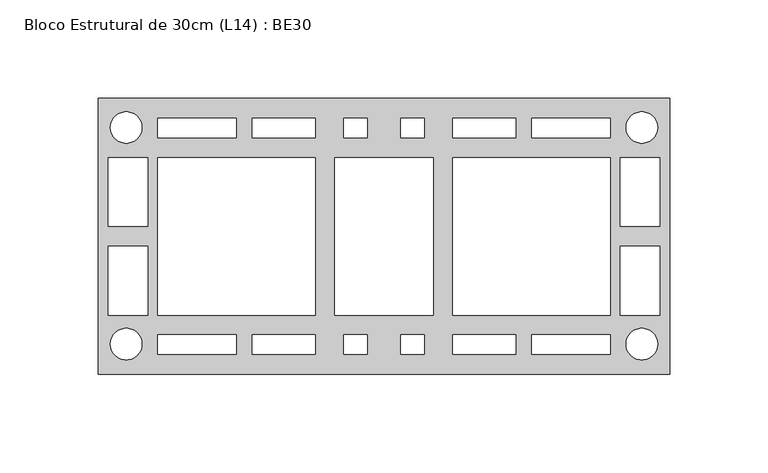
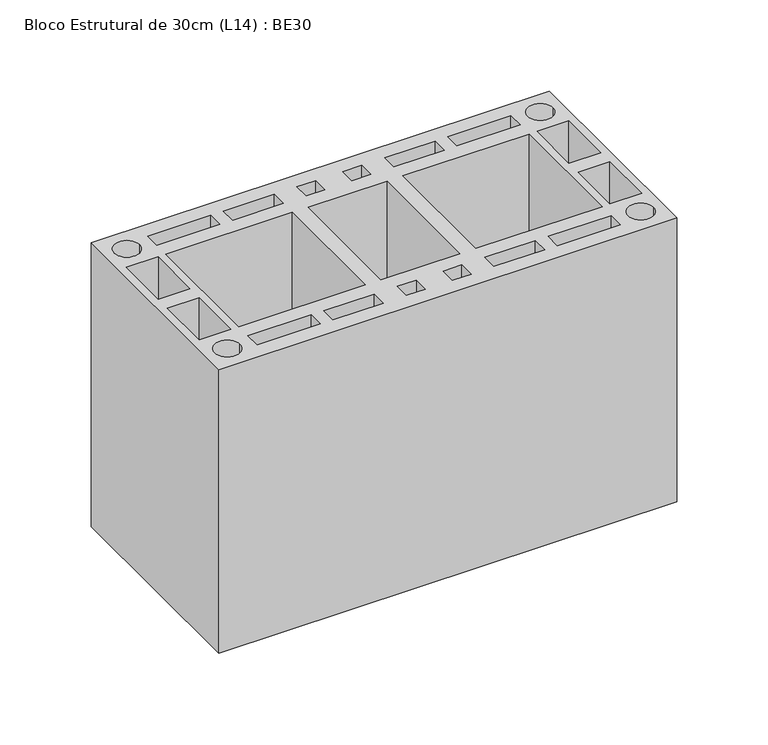
"""IFC4 building model written with IfcOpenShell, lengths in millimetres: proxy geometry, Bloco Estrutural de 30cm (L14) : BE30."""

from ifc_helpers import new_model, si_unit, point, frame_2d, origin, origin_with_axes, place, context, project, spatial, polyline, circle_curve, trimmed, segment, composite_curve, outline, extrude, source, transform, mapped, element, save


def bloco_estrutural_de_30cm_l14_be30_ec04c00f(model_context):
    return source(origin(), model_context, "Body", "SweptSolid", [
        extrude(outline(polyline([(290.0, 0.0), (290.0, -140.0), (0.0, -140.0), (0.0, 0.0), (290.0, 0.0)]), holes=[composite_curve([segment(trimmed(circle_curve(frame_2d((14.1087523, -124.7509514)), 8.0), [point((6.1087523, -124.7509514))], [point((22.1087523, -124.7509514))], True, "CARTESIAN"), True, "CONTINUOUS"), segment(trimmed(circle_curve(frame_2d((14.1087523, -124.7509514)), 8.0), [point((22.1087523, -124.7509514))], [point((6.1087523, -124.7509514))], True, "CARTESIAN"), True, "CONTINUOUS")], self_intersect=False), composite_curve([segment(trimmed(circle_curve(frame_2d((14.1087523, -14.7509514)), 8.0), [point((6.1087523, -14.7509514))], [point((22.1087523, -14.7509514))], True, "CARTESIAN"), True, "CONTINUOUS"), segment(trimmed(circle_curve(frame_2d((14.1087523, -14.7509514)), 8.0), [point((22.1087523, -14.7509514))], [point((6.1087523, -14.7509514))], True, "CARTESIAN"), True, "CONTINUOUS")], self_intersect=False), polyline([(110.0, -110.0), (110.0, -30.0), (30.0, -30.0), (30.0, -110.0), (110.0, -110.0)]), polyline([(170.0, -110.0), (170.0, -30.0), (120.0, -30.0), (120.0, -110.0), (170.0, -110.0)]), polyline([(70.0, -130.0), (70.0, -120.0), (30.0, -120.0), (30.0, -130.0), (70.0, -130.0)]), polyline([(70.0, -20.0), (70.0, -10.0), (30.0, -10.0), (30.0, -20.0), (70.0, -20.0)]), polyline([(78.0, -130.0), (110.0, -130.0), (110.0, -120.0), (78.0, -120.0), (78.0, -130.0)]), polyline([(78.0, -20.0), (110.0, -20.0), (110.0, -10.0), (78.0, -10.0), (78.0, -20.0)]), composite_curve([segment(trimmed(circle_curve(frame_2d((275.8912477, -124.7509514)), 8.0), [point((283.8912477, -124.7509514))], [point((267.8912477, -124.7509514))], True, "CARTESIAN"), True, "CONTINUOUS"), segment(trimmed(circle_curve(frame_2d((275.8912477, -124.7509514)), 8.0), [point((267.8912477, -124.7509514))], [point((283.8912477, -124.7509514))], True, "CARTESIAN"), True, "CONTINUOUS")], self_intersect=False), composite_curve([segment(trimmed(circle_curve(frame_2d((275.8912477, -14.7509514)), 8.0), [point((283.8912477, -14.7509514))], [point((267.8912477, -14.7509514))], True, "CARTESIAN"), True, "CONTINUOUS"), segment(trimmed(circle_curve(frame_2d((275.8912477, -14.7509514)), 8.0), [point((267.8912477, -14.7509514))], [point((283.8912477, -14.7509514))], True, "CARTESIAN"), True, "CONTINUOUS")], self_intersect=False), polyline([(180.0, -110.0), (260.0, -110.0), (260.0, -30.0), (180.0, -30.0), (180.0, -110.0)]), polyline([(220.0, -130.0), (260.0, -130.0), (260.0, -120.0), (220.0, -120.0), (220.0, -130.0)]), polyline([(220.0, -20.0), (260.0, -20.0), (260.0, -10.0), (220.0, -10.0), (220.0, -20.0)]), polyline([(212.0, -130.0), (212.0, -120.0), (180.0, -120.0), (180.0, -130.0), (212.0, -130.0)]), polyline([(212.0, -20.0), (212.0, -10.0), (180.0, -10.0), (180.0, -20.0), (212.0, -20.0)]), polyline([(25.0, -110.0), (25.0, -75.0), (5.0, -75.0), (5.0, -110.0), (25.0, -110.0)]), polyline([(25.0, -30.0), (5.0, -30.0), (5.0, -65.0), (25.0, -65.0), (25.0, -30.0)]), polyline([(265.0, -110.0), (285.0, -110.0), (285.0, -75.0), (265.0, -75.0), (265.0, -110.0)]), polyline([(265.0, -30.0), (265.0, -65.0), (285.0, -65.0), (285.0, -30.0), (265.0, -30.0)]), polyline([(153.5, -20.0), (165.5, -20.0), (165.5, -10.0), (153.5, -10.0), (153.5, -20.0)]), polyline([(136.5, -20.0), (136.5, -10.0), (124.5, -10.0), (124.5, -20.0), (136.5, -20.0)]), polyline([(153.5, -120.0), (153.5, -130.0), (165.5, -130.0), (165.5, -120.0), (153.5, -120.0)]), polyline([(136.5, -120.0), (124.5, -120.0), (124.5, -130.0), (136.5, -130.0), (136.5, -120.0)])]), origin_with_axes(), (0.0, 0.0, 1.0), 190.0),
    ])


if __name__ == "__main__":
    model = new_model("IFC4")
    model_context = context("Model", 3, world=origin())
    ifc_project = project(units=[si_unit("LENGTHUNIT", "METRE", prefix="MILLI")], contexts=[model_context])
    site = spatial("IfcSite", under=ifc_project)
    building = spatial("IfcBuilding", under=site)
    placement = place(None, origin())
    bloco_estrutural_de_30cm_l14_be30_shape = bloco_estrutural_de_30cm_l14_be30_ec04c00f(model_context)
    element("IfcBuildingElementProxy", 1, Name="Bloco Estrutural de 30cm (L14) : BE30", ObjectType="Bloco Estrutural de 30cm (L14) : BE30", at=placement, inside=building, context=model_context, shape_type="MappedRepresentation", body=[
        mapped(bloco_estrutural_de_30cm_l14_be30_shape, transform((0.0, 0.0, 0.0), x_axis=(1.0, 0.0, 0.0), y_axis=(0.0, 1.0, 0.0), z_axis=(0.0, 0.0, 1.0))),
    ])
    save(model, "model.ifc")

# Revit data of these elements
# Type "Bloco Estrutural de 30cm (L14) : BE30"
#   Material [instance default] = Blocos Cerâmicos
#   Default Elevation = 0
# Element 1 (IfcBuildingElementProxy, "Bloco Estrutural de 30cm (L14) : BE30")
#   Materials on its faces: "Blocos Cerâmicos"
# Materials
#   "Blocos Cerâmicos": class "Genérico", colour RGB 177 84 47, transparency 0, Cost = 0
